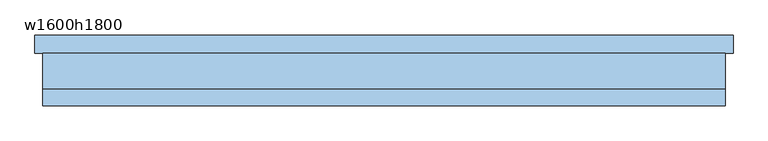
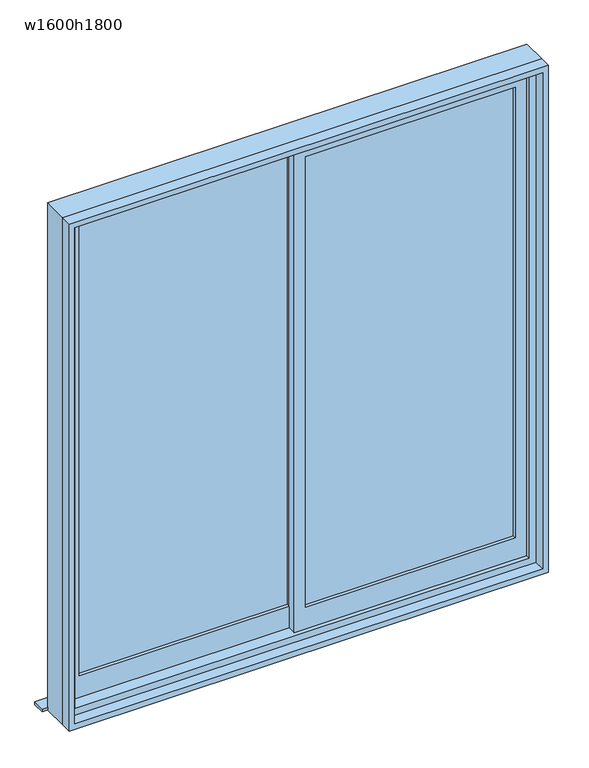
"""IFC4 building model written with IfcOpenShell, lengths in millimetres: window geometry, 引違い掃出窓_2枚 : w1600h1800."""

import ifcopenshell
import ifcopenshell.guid

model = None  # the IFC model being written
_history = None  # IfcOwnerHistory: only IFC2X3 demands one
_inside = {}  # id of a spatial element -> (the spatial element, [elements in it])
_under = {}  # id of a project, library or spatial element -> (it, [spatial elements below it])
_declared = {}  # id of a project -> (the project, [libraries it declares])
_typed = {}  # id of a type object -> (the type object, [elements of that type])
_made_of = {}  # id of a material, layer set ... -> (it, [elements and type objects made of it])


def new_model(schema):
    """Start an empty IFC model of exactly this schema.

    Asked for "IFC4X3", IfcOpenShell would pick the latest addendum, in which some entities
    have other attributes; the version numbers below select the first issue.
    IFC2X3 requires an IfcOwnerHistory on every rooted entity: one is made here for all.
    """
    global model, _history
    if schema == "IFC4X3":
        model = ifcopenshell.file(schema_version=(4, 3, 0, 0))
    else:
        model = ifcopenshell.file(schema=schema)
    _inside.clear()
    _under.clear()
    _declared.clear()
    _typed.clear()
    _made_of.clear()
    _history = None
    if model.schema == "IFC2X3":
        org = make("IfcOrganization", Name="unknown")
        user = make(
            "IfcPersonAndOrganization",
            ThePerson=make("IfcPerson", FamilyName="unknown"),
            TheOrganization=org,
        )
        app = make(
            "IfcApplication",
            ApplicationDeveloper=org,
            Version="unknown",
            ApplicationFullName="unknown",
            ApplicationIdentifier="unknown",
        )
        _history = make(
            "IfcOwnerHistory",
            OwningUser=user,
            OwningApplication=app,
            ChangeAction="ADDED",
            CreationDate=0,
        )
    return model


def make(cls, **values):
    """One entity of the class cls with the attributes given. An attribute that is None is left unset."""
    return model.create_entity(
        cls, **{name: value for name, value in values.items() if value is not None}
    )


def rooted(cls, **values):
    """An entity with a GlobalId (a new one), such as an element, a storey or a relation."""
    return make(cls, GlobalId=ifcopenshell.guid.new(), OwnerHistory=_history, **values)


def si_unit(unit_type, name, prefix=None):
    """IfcSIUnit, for example si_unit("LENGTHUNIT", "METRE", prefix="MILLI")."""
    return make("IfcSIUnit", UnitType=unit_type, Prefix=prefix, Name=name)


def assignment(units):
    """IfcUnitAssignment: the units of a project."""
    return None if units is None else make("IfcUnitAssignment", Units=units)


def point(xyz):
    """IfcCartesianPoint."""
    return None if xyz is None else make("IfcCartesianPoint", Coordinates=xyz)


def direction(xyz):
    """IfcDirection."""
    return None if xyz is None else make("IfcDirection", DirectionRatios=xyz)


def frame(location, z_axis=None, x_axis=None):
    """IfcAxis2Placement3D, a coordinate frame: its origin and axes. An axis left out is left unset."""
    return make(
        "IfcAxis2Placement3D",
        Location=point(location),
        Axis=direction(z_axis),
        RefDirection=direction(x_axis),
    )


def origin():
    """The frame at (0, 0, 0) with its axes left unset."""
    return frame((0.0, 0.0, 0.0))


def place(relative_to, where):
    """IfcLocalPlacement: puts the frame where relative to a parent placement (None: the world)."""
    return make(
        "IfcLocalPlacement", PlacementRelTo=relative_to, RelativePlacement=where
    )


def context(
    kind, dimensions, precision=None, world=None, true_north=None, identifier=None
):
    """IfcGeometricRepresentationContext, for example the 3D "Model" context."""
    return make(
        "IfcGeometricRepresentationContext",
        ContextIdentifier=identifier,
        ContextType=kind,
        CoordinateSpaceDimension=dimensions,
        Precision=precision,
        WorldCoordinateSystem=world,
        TrueNorth=true_north,
    )


def project(units=None, contexts=None):
    """IfcProject with its units and contexts."""
    return rooted(
        "IfcProject",
        Name="project",
        RepresentationContexts=contexts,
        UnitsInContext=assignment(units),
    )


def spatial(cls, under=None, at=None, **own):
    """A site, building, storey or space (cls), placed at a placement, below another one or the project."""
    s = rooted(cls, ObjectPlacement=at, **own)
    if under is not None:
        _under.setdefault(under.id(), (under, []))[1].append(s)
    return s


def polyline(points):
    """IfcPolyline through the points."""
    return make("IfcPolyline", Points=[point(p) for p in points])


def outline(outer, holes=None, kind="AREA"):
    """IfcArbitraryClosedProfileDef: a profile drawn as a closed curve; with holes, ...WithVoids."""
    if holes is None:
        return make("IfcArbitraryClosedProfileDef", ProfileType=kind, OuterCurve=outer)
    return make(
        "IfcArbitraryProfileDefWithVoids",
        ProfileType=kind,
        OuterCurve=outer,
        InnerCurves=holes,
    )


def extrude(swept, where, along, depth):
    """IfcExtrudedAreaSolid: the profile swept, set in the frame where, extruded along a direction by depth."""
    return make(
        "IfcExtrudedAreaSolid",
        SweptArea=swept,
        Position=where,
        ExtrudedDirection=direction(along),
        Depth=depth,
    )


def shape(context_of_items, identifier, shape_type, items):
    """IfcShapeRepresentation: the items that make up one representation, for example the "Body"."""
    return make(
        "IfcShapeRepresentation",
        ContextOfItems=context_of_items,
        RepresentationIdentifier=identifier,
        RepresentationType=shape_type,
        Items=items,
    )


def source(mapping_origin, context_of_items, identifier, shape_type, items):
    """IfcRepresentationMap: a shape defined once, which mapped items show again and again."""
    return make(
        "IfcRepresentationMap",
        MappingOrigin=mapping_origin,
        MappedRepresentation=shape(context_of_items, identifier, shape_type, items),
    )


def transform(
    local_origin,
    x_axis=None,
    y_axis=None,
    z_axis=None,
    scale=None,
    scale2=None,
    scale3=None,
    uniform=True,
):
    """IfcCartesianTransformationOperator3D, or its non-uniform kind. x_axis, y_axis, z_axis: its Axis1, 2, 3."""
    if uniform:
        return make(
            "IfcCartesianTransformationOperator3D",
            Axis1=direction(x_axis),
            Axis2=direction(y_axis),
            LocalOrigin=point(local_origin),
            Scale=scale,
            Axis3=direction(z_axis),
        )
    return make(
        "IfcCartesianTransformationOperator3DnonUniform",
        Axis1=direction(x_axis),
        Axis2=direction(y_axis),
        LocalOrigin=point(local_origin),
        Scale=scale,
        Axis3=direction(z_axis),
        Scale2=scale2,
        Scale3=scale3,
    )


def mapped(mapping_source, mapping_target):
    """IfcMappedItem: shows the shape of a source again, moved by a transform."""
    return make(
        "IfcMappedItem", MappingSource=mapping_source, MappingTarget=mapping_target
    )


def made_of(thing, what):
    """Note that an element or type object is made of a material, layer set ...; save() writes the relation."""
    if what is not None:
        _made_of.setdefault(what.id(), (what, []))[1].append(thing)
    return thing


def element(
    cls,
    number,
    at=None,
    inside=None,
    cuts=None,
    type_object=None,
    material=None,
    context=None,
    identifier="Body",
    shape_type=None,
    held_by="IfcProductDefinitionShape",
    body=None,
    shapes=None,
    **own,
):
    """One element of the class cls, such as IfcWall. Its Tag is "e" and its number.

    at: its placement. inside: the storey or other place that contains it. cuts: it is an
    opening in that element (IfcRelVoidsElement). A single representation is given by context,
    identifier, shape_type and body (its items); several are given by shapes. held_by: the class
    of the entity that holds the representations. save() writes the other relations.
    """
    e = rooted(cls, Tag="e%d" % number, ObjectPlacement=at, **own)
    if body is not None:
        shapes = [shape(context, identifier, shape_type, body)]
    if shapes is not None:
        e.Representation = make(held_by, Representations=shapes)
    if inside is not None:
        _inside.setdefault(inside.id(), (inside, []))[1].append(e)
    if cuts is not None:
        rooted(
            "IfcRelVoidsElement", RelatingBuildingElement=cuts, RelatedOpeningElement=e
        )
    if type_object is not None:
        _typed.setdefault(type_object.id(), (type_object, []))[1].append(e)
    return made_of(e, material)


def aggregate(whole, parts):
    """IfcRelAggregates: a whole, such as a stair, and the parts it consists of."""
    return rooted("IfcRelAggregates", RelatingObject=whole, RelatedObjects=parts)


def save(model, path):
    """Write the relations noted so far, then the file.

    IfcRelAggregates (storeys below a building ...), IfcRelContainedInSpatialStructure (elements
    in a storey), IfcRelDefinesByType, IfcRelAssociatesMaterial and IfcRelDeclares: one each for
    every whole, place, type object, material and project.
    """
    for whole, parts in _under.values():
        aggregate(whole, parts)
    for where, things in _inside.values():
        rooted(
            "IfcRelContainedInSpatialStructure",
            RelatedElements=things,
            RelatingStructure=where,
        )
    for kind, things in _typed.values():
        rooted("IfcRelDefinesByType", RelatedObjects=things, RelatingType=kind)
    for what, things in _made_of.values():
        rooted("IfcRelAssociatesMaterial", RelatedObjects=things, RelatingMaterial=what)
    for by, libraries in _declared.values():
        rooted("IfcRelDeclares", RelatingContext=by, RelatedDefinitions=libraries)
    model.write(path)


def w1600h1800_bd36f67d(model_context):
    return source(origin(), model_context, "Body", "SweptSolid", [
        extrude(outline(polyline([(-20.0, 12.5), (-760.0, 12.5), (-760.0, 17.5), (-20.0, 17.5), (-20.0, 12.5)])), frame((0.0, 0.0, 280.0), z_axis=(0.0, 0.0, 1.0), x_axis=(1.0, 0.0, 0.0)), (0.0, 0.0, 1.0), 1680.0),
        extrude(outline(polyline([(760.0, -17.5), (20.0, -17.5), (20.0, -12.5), (760.0, -12.5), (760.0, -17.5)])), frame((0.0, 0.0, 280.0), z_axis=(0.0, 0.0, 1.0), x_axis=(1.0, 0.0, 0.0)), (0.0, 0.0, 1.0), 1680.0),
        extrude(outline(polyline([(2000.0, -20.0), (200.0, -20.0), (200.0, 800.0), (2000.0, 800.0), (2000.0, -20.0)]), holes=[polyline([(280.0, 760.0), (280.0, 20.0), (1960.0, 20.0), (1960.0, 760.0), (280.0, 760.0)])]), frame((0.0, -30.0, 0.0), z_axis=(0.0, 1.0, 0.0), x_axis=(0.0, 0.0, 1.0)), (0.0, 0.0, 1.0), 30.0),
        extrude(outline(polyline([(2000.0, -800.0), (200.0, -800.0), (200.0, 20.0), (2000.0, 20.0), (2000.0, -800.0)]), holes=[polyline([(280.0, -20.0), (280.0, -760.0), (1960.0, -760.0), (1960.0, -20.0), (280.0, -20.0)])]), frame((0.0, 0.0, 0.0), z_axis=(0.0, 1.0, 0.0), x_axis=(0.0, 0.0, 1.0)), (0.0, 0.0, 1.0), 30.0),
        extrude(outline(polyline([(865.0, 90.0), (865.0, 45.0), (-865.0, 45.0), (-865.0, 90.0), (865.0, 90.0)])), frame((0.0, 0.0, 155.0), z_axis=(0.0, 0.0, 1.0), x_axis=(1.0, 0.0, 0.0)), (0.0, 0.0, 1.0), 10.0),
        extrude(outline(polyline([(2045.0, 845.0), (2045.0, -845.0), (155.0, -845.0), (155.0, 845.0), (2045.0, 845.0)]), holes=[polyline([(175.0, -825.0), (2025.0, -825.0), (2025.0, 825.0), (175.0, 825.0), (175.0, -825.0)])]), frame((0.0, -85.0, 0.0), z_axis=(0.0, 1.0, 0.0), x_axis=(0.0, 0.0, 1.0)), (0.0, 0.0, 1.0), 40.0),
        extrude(outline(polyline([(2045.0, -845.0), (155.0, -845.0), (155.0, 845.0), (2045.0, 845.0), (2045.0, -845.0)]), holes=[polyline([(2000.0, 800.0), (200.0, 800.0), (200.0, -800.0), (2000.0, -800.0), (2000.0, 800.0)])]), frame((0.0, -45.0, 0.0), z_axis=(0.0, 1.0, 0.0), x_axis=(0.0, 0.0, 1.0)), (0.0, 0.0, 1.0), 90.0),
    ])


if __name__ == "__main__":
    model = new_model("IFC4")
    model_context = context("Model", 3, world=origin())
    ifc_project = project(units=[si_unit("LENGTHUNIT", "METRE", prefix="MILLI")], contexts=[model_context])
    site = spatial("IfcSite", under=ifc_project)
    building = spatial("IfcBuilding", under=site)
    placement = place(None, origin())
    w1600h1800_shape = w1600h1800_bd36f67d(model_context)
    element("IfcWindow", 1, ObjectType="引違い掃出窓_2枚 : w1600h1800", at=placement, inside=building, context=model_context, shape_type="MappedRepresentation", body=[
        mapped(w1600h1800_shape, transform((0.0, 0.0, 0.0), x_axis=(1.0, 0.0, 0.0), y_axis=(0.0, 1.0, 0.0), z_axis=(0.0, 0.0, 1.0))),
    ])
    save(model, "model.ifc")

# Revit data of these elements
# Project information
#   プロジェクト発行日 = "発行日"
#   プロジェクト ステータス = "プロジェクト ステータス"
#   クライアント名 = "オーナ"
#   計画地住所 = "ここにアドレスを入力"
#   プロジェクト名 = "プロジェクト名"
#   プロジェクト番号 = "0001"
# Type "引違い掃出窓_2枚 : w1600h1800"
#   Construction Type Id = "GSP4R"
#   Analytic Construction = "1/8 インチ ピルキントン一重ガラス"
#   Type Mark = "67"
#   Operation = "ダブル パネル縦"
#   Keynote = "08520.R1"
#   Visual Light Transmittance = 0.9
#   Solar Heat Gain Coefficient = 0.86
#   Heat Transfer Coefficient (U) = 6.7069 W/(m²·K)
#   Height = 1800 mm
#   既定の腰高 = 200 mm
#   Width = 1600 mm
#   額縁見附 = 20 mm
#   額縁ちり = 10 mm
#   サッシ見附 = 45 mm
#   サッシの幅 = 90 mm
#   サッシ額縁 [instance default] = none
#   サッシ本体 [instance default] = none
#   サッシガラス [instance default] = ガラス - 透明
#   Manufacturer = ""
#   Wall Closure = (empty or 0)
#   Model = ""
#   Type Comments = ""
#   Assembly Code = ""
# Element 1 (IfcWindow, "引違い掃出窓_2枚 : w1600h1800")
#   Materials on its faces: "ガラス - 透明"
# Materials
#   "ガラス - 透明": class "ガラス", colour RGB 0 128 192, transparency 0.9, Cost = 0
